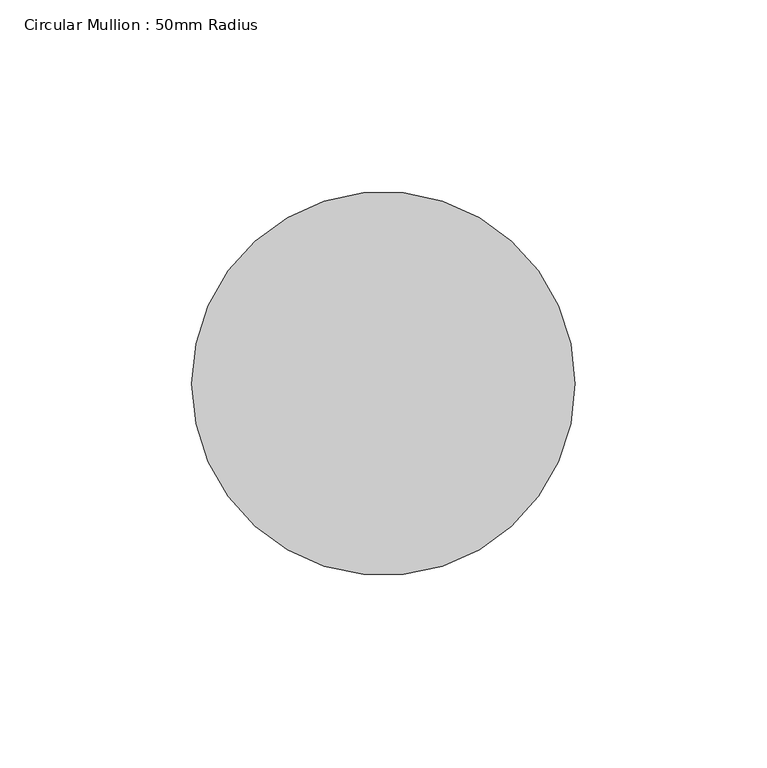
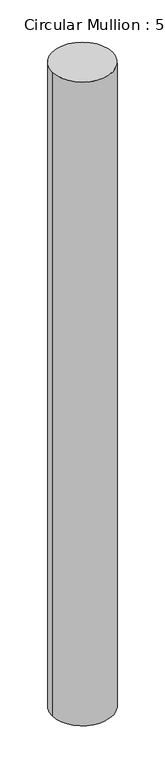
"""IFC4 building model written with IfcOpenShell, lengths in millimetres: member geometry, Circular Mullion : 50mm Radius."""

from ifc_helpers import new_model, si_unit, point, frame, origin, origin_2d, place, context, project, spatial, circle_curve, trimmed, segment, composite_curve, outline, extrude, source, transform, mapped, element, save


def circular_mullion_50mm_radius_fe642d66(model_context):
    return source(origin(), model_context, "Body", "SweptSolid", [
        extrude(outline(composite_curve([segment(trimmed(circle_curve(origin_2d(), 50.0), [point((50.0, 0.0))], [point((-50.0, 0.0))], False, "CARTESIAN"), True, "CONTINUOUS"), segment(trimmed(circle_curve(origin_2d(), 50.0), [point((-50.0, 0.0))], [point((50.0, 0.0))], False, "CARTESIAN"), True, "CONTINUOUS")], self_intersect=False)), frame((0.0, 0.0, -1130.2651221), z_axis=(0.0, 0.0, 1.0), x_axis=(1.0, 0.0, 0.0)), (0.0, 0.0, 1.0), 1130.2651221),
    ])


if __name__ == "__main__":
    model = new_model("IFC4")
    model_context = context("Model", 3, world=origin())
    ifc_project = project(units=[si_unit("LENGTHUNIT", "METRE", prefix="MILLI")], contexts=[model_context])
    site = spatial("IfcSite", under=ifc_project)
    building = spatial("IfcBuilding", under=site)
    placement = place(None, origin())
    circular_mullion_50mm_radius_shape = circular_mullion_50mm_radius_fe642d66(model_context)
    element("IfcMember", 1, ObjectType="Circular Mullion : 50mm Radius", at=placement, inside=building, context=model_context, shape_type="MappedRepresentation", body=[
        mapped(circular_mullion_50mm_radius_shape, transform((0.0, 0.0, 0.0), x_axis=(1.0, 0.0, 0.0), y_axis=(0.0, 1.0, 0.0), z_axis=(0.0, 0.0, 1.0))),
    ])
    save(model, "model.ifc")

# Revit data of these elements
# Type "Circular Mullion : 50mm Radius"
#   built-in parameter 1007350 = 0.164042 (stored number, unit not read)
# Element 1 (IfcMember, "Circular Mullion : 50mm Radius")
#   Materials on its faces: "Aluminium"
# Materials
#   "Aluminium": class "Metal", colour RGB 247 247 247, transparency 0, Description = "Aluminium 6061", Cost = 0
